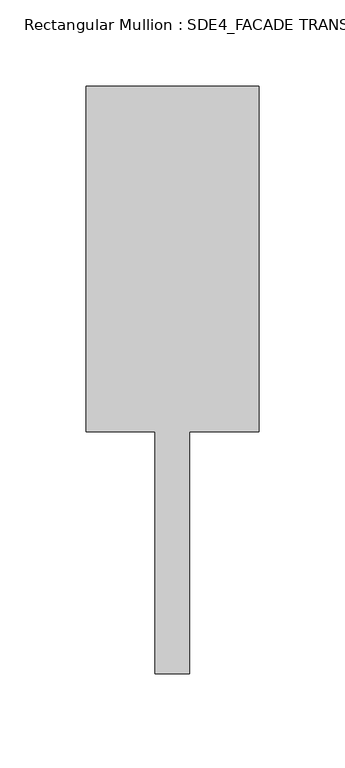
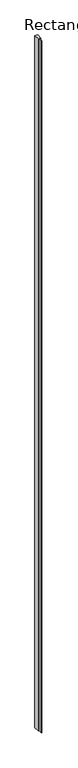
"""IFC4 building model written with IfcOpenShell, lengths in millimetres: member geometry, Rectangular Mullion : SDE4_FACADE TRANSOM TYPE 1."""

from ifc_helpers import new_model, si_unit, frame, origin, place, context, project, spatial, polyline, outline, extrude, source, transform, mapped, element, save


def rectangular_mullion_sde4_facade_transom_type_1_ddc89f88(model_context):
    return source(origin(), model_context, "Body", "SweptSolid", [
        extrude(outline(polyline([(50.0, 132.5), (50.0, -67.5), (10.0, -67.5), (10.0, -207.5), (-10.0, -207.5), (-10.0, -67.5), (-50.0, -67.5), (-50.0, 132.5), (50.0, 132.5)])), frame((0.0, 0.0, -26676.2995218), z_axis=(0.0, 0.0, 1.0), x_axis=(1.0, 0.0, 0.0)), (0.0, 0.0, 1.0), 26676.2995218),
    ])


if __name__ == "__main__":
    model = new_model("IFC4")
    model_context = context("Model", 3, world=origin())
    ifc_project = project(units=[si_unit("LENGTHUNIT", "METRE", prefix="MILLI")], contexts=[model_context])
    site = spatial("IfcSite", under=ifc_project)
    building = spatial("IfcBuilding", under=site)
    placement = place(None, origin())
    rectangular_mullion_sde4_facade_transom_type_1_shape = rectangular_mullion_sde4_facade_transom_type_1_ddc89f88(model_context)
    element("IfcMember", 1, ObjectType="Rectangular Mullion : SDE4_FACADE TRANSOM TYPE 1", at=placement, inside=building, context=model_context, shape_type="MappedRepresentation", body=[
        mapped(rectangular_mullion_sde4_facade_transom_type_1_shape, transform((0.0, 0.0, 0.0), x_axis=(1.0, 0.0, 0.0), y_axis=(0.0, 1.0, 0.0), z_axis=(0.0, 0.0, 1.0))),
    ])
    save(model, "model.ifc")

# Revit data of these elements
# Type "Rectangular Mullion : SDE4_FACADE TRANSOM TYPE 1"
#   built-in parameter 1007322 = 1.11549 (stored number, unit not read)
#   built-in parameter 1007321 = 0.164042 (stored number, unit not read)
#   built-in parameter 1007320 = 0.164042 (stored number, unit not read)
